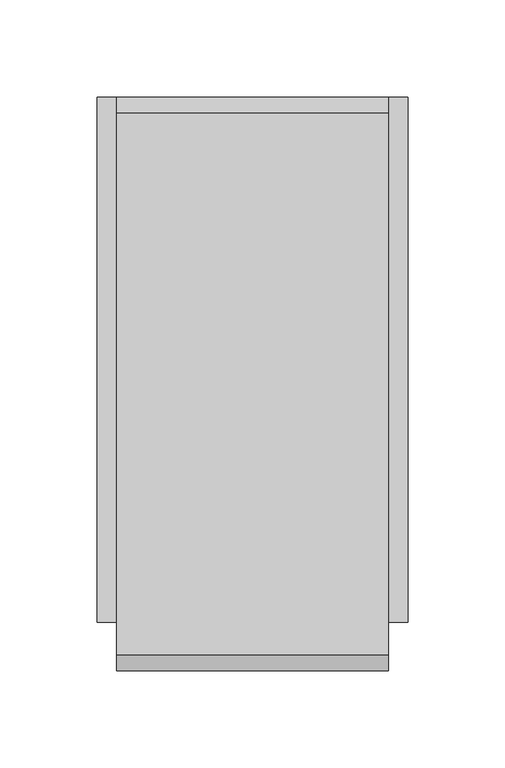
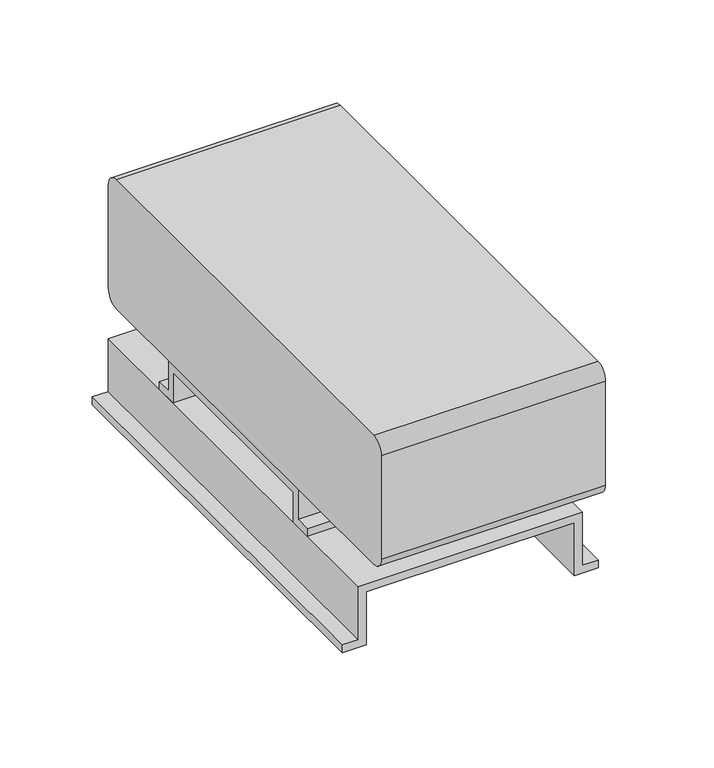
"""IFC4 building model written with IfcOpenShell, lengths in millimetres: proxy geometry, ВЕЗА_КПУ-1Н_ЭП230В : ВЕЗА_КПУ-1Н_ЭП230В."""

from ifc_helpers import new_model, si_unit, point, frame, frame_2d, origin, place, context, project, spatial, polyline, circle_curve, trimmed, segment, composite_curve, outline, extrude, source, transform, mapped, element, save


def mechanical_equipment_c2249724(model_context):
    return source(origin(), model_context, "Body", "SweptSolid", [
        extrude(outline(composite_curve([segment(polyline([(135.0, 141.6473986), (135.0, 73.444316)]), True, "CONTINUOUS"), segment(trimmed(circle_curve(frame_2d((126.555684, 73.444316)), 8.444316), [point((135.0, 73.444316))], [point((126.555684, 65.0))], False, "CARTESIAN"), True, "CONTINUOUS"), segment(polyline([(126.555684, 65.0), (-151.8441775, 65.0)]), True, "CONTINUOUS"), segment(trimmed(circle_curve(frame_2d((-151.8441775, 73.1558225)), 8.1558225), [point((-151.8441775, 65.0))], [point((-160.0, 73.1558225))], False, "CARTESIAN"), True, "CONTINUOUS"), segment(polyline([(-160.0, 73.1558225), (-160.0, 141.668104)]), True, "CONTINUOUS"), segment(trimmed(circle_curve(frame_2d((-151.668104, 141.668104)), 8.331896), [point((-160.0, 141.668104))], [point((-151.668104, 150.0))], False, "CARTESIAN"), True, "CONTINUOUS"), segment(polyline([(-151.668104, 150.0), (126.6473986, 150.0)]), True, "CONTINUOUS"), segment(trimmed(circle_curve(frame_2d((126.6473986, 141.6473986)), 8.3526014), [point((126.6473986, 150.0))], [point((135.0, 141.6473986))], False, "CARTESIAN"), True, "CONTINUOUS")], self_intersect=False)), frame((-70.0, 0.0, 0.0), z_axis=(1.0, 0.0, 0.0), x_axis=(0.0, 1.0, 0.0)), (0.0, 0.0, 1.0), 140.0),
        extrude(outline(polyline([(-80.0, 40.0), (-80.0, 45.0), (-70.0, 45.0), (-70.0, 65.0), (70.0, 65.0), (70.0, 45.0), (80.0, 45.0), (80.0, 40.0), (65.0, 40.0), (65.0, 60.0), (-65.0, 60.0), (-65.0, 40.0), (-80.0, 40.0)])), frame((-70.0, 0.0, 0.0), z_axis=(1.0, 0.0, 0.0), x_axis=(0.0, 1.0, 0.0)), (0.0, 0.0, 1.0), 140.0),
        extrude(outline(polyline([(0.0, -80.0), (0.0, -65.0), (35.0, -65.0), (35.0, 65.0), (0.0, 65.0), (0.0, 80.0), (5.0, 80.0), (5.0, 70.0), (40.0, 70.0), (40.0, -70.0), (5.0, -70.0), (5.0, -80.0), (0.0, -80.0)])), frame((0.0, -135.0, 0.0), z_axis=(0.0, 1.0, 0.0), x_axis=(0.0, 0.0, 1.0)), (0.0, 0.0, 1.0), 270.0),
    ])


if __name__ == "__main__":
    model = new_model("IFC4")
    model_context = context("Model", 3, world=origin())
    ifc_project = project(units=[si_unit("LENGTHUNIT", "METRE", prefix="MILLI")], contexts=[model_context])
    site = spatial("IfcSite", under=ifc_project)
    building = spatial("IfcBuilding", under=site)
    placement = place(None, origin())
    mechanical_equipment_shape = mechanical_equipment_c2249724(model_context)
    element("IfcBuildingElementProxy", 1, Name="ВЕЗА_КПУ-1Н_ЭП230В : ВЕЗА_КПУ-1Н_ЭП230В", ObjectType="ВЕЗА_КПУ-1Н_ЭП230В : ВЕЗА_КПУ-1Н_ЭП230В", at=placement, inside=building, context=model_context, shape_type="MappedRepresentation", body=[
        mapped(mechanical_equipment_shape, transform((0.0, 0.0, 0.0), x_axis=(1.0, 0.0, 0.0), y_axis=(0.0, 1.0, 0.0), z_axis=(0.0, 0.0, 1.0))),
    ])
    save(model, "model.ifc")

# Revit data of these elements
# Type "ВЕЗА_КПУ-1Н_ЭП230В : ВЕЗА_КПУ-1Н_ЭП230В"
#   ВЕЗА_Контакты = "bim@veza.ru"
#   ВЕЗА_Классификатор = ""
#   ADSK_Примечание = "!Не учитывать"
#   ADSK_Позиция = ""
#   ADSK_Наименование краткое = ""
#   ADSK_Наименование = "Электропривод"
#   ADSK_Марка [instance default] = ""
#   ADSK_Комплект [instance default] = ""
#   ADSK_Код изделия = ""
#   ADSK_Завод-изготовитель = "ООО ''ВЕЗА''"
#   ADSK_Единица измерения = "шт."
#   ADSK_Группирование = ""
#   Ширина рукоятки = 30 mm
#   Ширина короба = 70 mm
#   Ширина = 130 mm
#   Расстояние до основания = 40 mm
#   Default Elevation = 1219.2 mm
#   Длина рукоятки = 84.866 mm
#   Длина отступ = 60 mm
#   Длина = 270 mm
#   H [instance default] = 170 mm
#   ADSK_Напряжение [instance default] = 230 V
#   ADSK_Масса = 0
#   ADSK_Количество = 1
#   Материал рукоятка = ВЕЗА_Резина
#   Материал модуль = ВЕЗА_Пластик
#   Материал деталь = ВЕЗА_Поверхность_Красная
#   Материал = none
# Element 1 (IfcBuildingElementProxy, "ВЕЗА_КПУ-1Н_ЭП230В : ВЕЗА_КПУ-1Н_ЭП230В")
#   H = 150 mm
#   Materials on its faces: "ВЕЗА_Поверхность_Красная"
# Materials
#   "ВЕЗА_Резина": class "Типовые", colour RGB 26 68 215, transparency 0, Cost = 0
#   "ВЕЗА_Пластик": class "Типовые", colour RGB 120 120 120, transparency 0, Cost = 0
#   "ВЕЗА_Поверхность_Красная": class "Metal", colour RGB 255 0 0, transparency 0, Description = "Сталь окрашенная", Cost = 0
